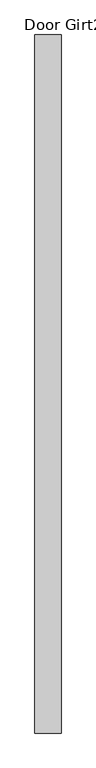
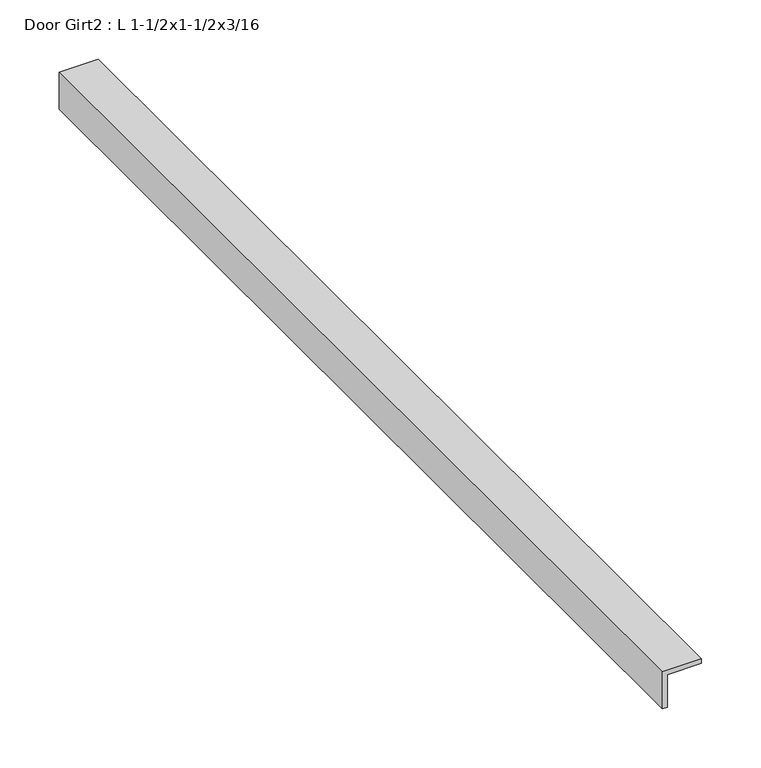
"""IFC4 building model written with IfcOpenShell, lengths in millimetres: proxy geometry, Door Girt2 : L 1-1/2x1-1/2x3/16."""

import ifcopenshell
import ifcopenshell.guid

model = None  # the IFC model being written
_history = None  # IfcOwnerHistory: only IFC2X3 demands one
_inside = {}  # id of a spatial element -> (the spatial element, [elements in it])
_under = {}  # id of a project, library or spatial element -> (it, [spatial elements below it])
_declared = {}  # id of a project -> (the project, [libraries it declares])
_typed = {}  # id of a type object -> (the type object, [elements of that type])
_made_of = {}  # id of a material, layer set ... -> (it, [elements and type objects made of it])


def new_model(schema):
    """Start an empty IFC model of exactly this schema.

    Asked for "IFC4X3", IfcOpenShell would pick the latest addendum, in which some entities
    have other attributes; the version numbers below select the first issue.
    IFC2X3 requires an IfcOwnerHistory on every rooted entity: one is made here for all.
    """
    global model, _history
    if schema == "IFC4X3":
        model = ifcopenshell.file(schema_version=(4, 3, 0, 0))
    else:
        model = ifcopenshell.file(schema=schema)
    _inside.clear()
    _under.clear()
    _declared.clear()
    _typed.clear()
    _made_of.clear()
    _history = None
    if model.schema == "IFC2X3":
        org = make("IfcOrganization", Name="unknown")
        user = make(
            "IfcPersonAndOrganization",
            ThePerson=make("IfcPerson", FamilyName="unknown"),
            TheOrganization=org,
        )
        app = make(
            "IfcApplication",
            ApplicationDeveloper=org,
            Version="unknown",
            ApplicationFullName="unknown",
            ApplicationIdentifier="unknown",
        )
        _history = make(
            "IfcOwnerHistory",
            OwningUser=user,
            OwningApplication=app,
            ChangeAction="ADDED",
            CreationDate=0,
        )
    return model


def make(cls, **values):
    """One entity of the class cls with the attributes given. An attribute that is None is left unset."""
    return model.create_entity(
        cls, **{name: value for name, value in values.items() if value is not None}
    )


def rooted(cls, **values):
    """An entity with a GlobalId (a new one), such as an element, a storey or a relation."""
    return make(cls, GlobalId=ifcopenshell.guid.new(), OwnerHistory=_history, **values)


def si_unit(unit_type, name, prefix=None):
    """IfcSIUnit, for example si_unit("LENGTHUNIT", "METRE", prefix="MILLI")."""
    return make("IfcSIUnit", UnitType=unit_type, Prefix=prefix, Name=name)


def assignment(units):
    """IfcUnitAssignment: the units of a project."""
    return None if units is None else make("IfcUnitAssignment", Units=units)


def point(xyz):
    """IfcCartesianPoint."""
    return None if xyz is None else make("IfcCartesianPoint", Coordinates=xyz)


def direction(xyz):
    """IfcDirection."""
    return None if xyz is None else make("IfcDirection", DirectionRatios=xyz)


def frame(location, z_axis=None, x_axis=None):
    """IfcAxis2Placement3D, a coordinate frame: its origin and axes. An axis left out is left unset."""
    return make(
        "IfcAxis2Placement3D",
        Location=point(location),
        Axis=direction(z_axis),
        RefDirection=direction(x_axis),
    )


def origin():
    """The frame at (0, 0, 0) with its axes left unset."""
    return frame((0.0, 0.0, 0.0))


def place(relative_to, where):
    """IfcLocalPlacement: puts the frame where relative to a parent placement (None: the world)."""
    return make(
        "IfcLocalPlacement", PlacementRelTo=relative_to, RelativePlacement=where
    )


def context(
    kind, dimensions, precision=None, world=None, true_north=None, identifier=None
):
    """IfcGeometricRepresentationContext, for example the 3D "Model" context."""
    return make(
        "IfcGeometricRepresentationContext",
        ContextIdentifier=identifier,
        ContextType=kind,
        CoordinateSpaceDimension=dimensions,
        Precision=precision,
        WorldCoordinateSystem=world,
        TrueNorth=true_north,
    )


def project(units=None, contexts=None):
    """IfcProject with its units and contexts."""
    return rooted(
        "IfcProject",
        Name="project",
        RepresentationContexts=contexts,
        UnitsInContext=assignment(units),
    )


def spatial(cls, under=None, at=None, **own):
    """A site, building, storey or space (cls), placed at a placement, below another one or the project."""
    s = rooted(cls, ObjectPlacement=at, **own)
    if under is not None:
        _under.setdefault(under.id(), (under, []))[1].append(s)
    return s


def polyline(points):
    """IfcPolyline through the points."""
    return make("IfcPolyline", Points=[point(p) for p in points])


def outline(outer, holes=None, kind="AREA"):
    """IfcArbitraryClosedProfileDef: a profile drawn as a closed curve; with holes, ...WithVoids."""
    if holes is None:
        return make("IfcArbitraryClosedProfileDef", ProfileType=kind, OuterCurve=outer)
    return make(
        "IfcArbitraryProfileDefWithVoids",
        ProfileType=kind,
        OuterCurve=outer,
        InnerCurves=holes,
    )


def extrude(swept, where, along, depth):
    """IfcExtrudedAreaSolid: the profile swept, set in the frame where, extruded along a direction by depth."""
    return make(
        "IfcExtrudedAreaSolid",
        SweptArea=swept,
        Position=where,
        ExtrudedDirection=direction(along),
        Depth=depth,
    )


def shape(context_of_items, identifier, shape_type, items):
    """IfcShapeRepresentation: the items that make up one representation, for example the "Body"."""
    return make(
        "IfcShapeRepresentation",
        ContextOfItems=context_of_items,
        RepresentationIdentifier=identifier,
        RepresentationType=shape_type,
        Items=items,
    )


def source(mapping_origin, context_of_items, identifier, shape_type, items):
    """IfcRepresentationMap: a shape defined once, which mapped items show again and again."""
    return make(
        "IfcRepresentationMap",
        MappingOrigin=mapping_origin,
        MappedRepresentation=shape(context_of_items, identifier, shape_type, items),
    )


def transform(
    local_origin,
    x_axis=None,
    y_axis=None,
    z_axis=None,
    scale=None,
    scale2=None,
    scale3=None,
    uniform=True,
):
    """IfcCartesianTransformationOperator3D, or its non-uniform kind. x_axis, y_axis, z_axis: its Axis1, 2, 3."""
    if uniform:
        return make(
            "IfcCartesianTransformationOperator3D",
            Axis1=direction(x_axis),
            Axis2=direction(y_axis),
            LocalOrigin=point(local_origin),
            Scale=scale,
            Axis3=direction(z_axis),
        )
    return make(
        "IfcCartesianTransformationOperator3DnonUniform",
        Axis1=direction(x_axis),
        Axis2=direction(y_axis),
        LocalOrigin=point(local_origin),
        Scale=scale,
        Axis3=direction(z_axis),
        Scale2=scale2,
        Scale3=scale3,
    )


def mapped(mapping_source, mapping_target):
    """IfcMappedItem: shows the shape of a source again, moved by a transform."""
    return make(
        "IfcMappedItem", MappingSource=mapping_source, MappingTarget=mapping_target
    )


def made_of(thing, what):
    """Note that an element or type object is made of a material, layer set ...; save() writes the relation."""
    if what is not None:
        _made_of.setdefault(what.id(), (what, []))[1].append(thing)
    return thing


def element(
    cls,
    number,
    at=None,
    inside=None,
    cuts=None,
    type_object=None,
    material=None,
    context=None,
    identifier="Body",
    shape_type=None,
    held_by="IfcProductDefinitionShape",
    body=None,
    shapes=None,
    **own,
):
    """One element of the class cls, such as IfcWall. Its Tag is "e" and its number.

    at: its placement. inside: the storey or other place that contains it. cuts: it is an
    opening in that element (IfcRelVoidsElement). A single representation is given by context,
    identifier, shape_type and body (its items); several are given by shapes. held_by: the class
    of the entity that holds the representations. save() writes the other relations.
    """
    e = rooted(cls, Tag="e%d" % number, ObjectPlacement=at, **own)
    if body is not None:
        shapes = [shape(context, identifier, shape_type, body)]
    if shapes is not None:
        e.Representation = make(held_by, Representations=shapes)
    if inside is not None:
        _inside.setdefault(inside.id(), (inside, []))[1].append(e)
    if cuts is not None:
        rooted(
            "IfcRelVoidsElement", RelatingBuildingElement=cuts, RelatedOpeningElement=e
        )
    if type_object is not None:
        _typed.setdefault(type_object.id(), (type_object, []))[1].append(e)
    return made_of(e, material)


def aggregate(whole, parts):
    """IfcRelAggregates: a whole, such as a stair, and the parts it consists of."""
    return rooted("IfcRelAggregates", RelatingObject=whole, RelatedObjects=parts)


def save(model, path):
    """Write the relations noted so far, then the file.

    IfcRelAggregates (storeys below a building ...), IfcRelContainedInSpatialStructure (elements
    in a storey), IfcRelDefinesByType, IfcRelAssociatesMaterial and IfcRelDeclares: one each for
    every whole, place, type object, material and project.
    """
    for whole, parts in _under.values():
        aggregate(whole, parts)
    for where, things in _inside.values():
        rooted(
            "IfcRelContainedInSpatialStructure",
            RelatedElements=things,
            RelatingStructure=where,
        )
    for kind, things in _typed.values():
        rooted("IfcRelDefinesByType", RelatedObjects=things, RelatingType=kind)
    for what, things in _made_of.values():
        rooted("IfcRelAssociatesMaterial", RelatedObjects=things, RelatingMaterial=what)
    for by, libraries in _declared.values():
        rooted("IfcRelDeclares", RelatingContext=by, RelatedDefinitions=libraries)
    model.write(path)


def door_girt2_l_1_1_2x1_1_2x3_16_4184d8b8(model_context):
    return source(origin(), model_context, "Body", "SweptSolid", [
        extrude(outline(polyline([(812.8, 587403.9934739), (812.8, 587365.8934739), (774.7, 587365.8934739), (774.7, 587370.6559739), (808.0375, 587370.6559739), (808.0375, 587403.9934739), (812.8, 587403.9934739)])), frame((0.0, -535163.4663841, 0.0), z_axis=(0.0, 1.0, 0.0), x_axis=(0.0, 0.0, 1.0)), (0.0, 0.0, 1.0), 1017.5875),
    ])


if __name__ == "__main__":
    model = new_model("IFC4")
    model_context = context("Model", 3, world=origin())
    ifc_project = project(units=[si_unit("LENGTHUNIT", "METRE", prefix="MILLI")], contexts=[model_context])
    site = spatial("IfcSite", under=ifc_project)
    building = spatial("IfcBuilding", under=site)
    placement = place(None, origin())
    door_girt2_l_1_1_2x1_1_2x3_16_shape = door_girt2_l_1_1_2x1_1_2x3_16_4184d8b8(model_context)
    element("IfcBuildingElementProxy", 1, Name="Door Girt2 : L 1-1/2x1-1/2x3/16", ObjectType="Door Girt2 : L 1-1/2x1-1/2x3/16", at=placement, inside=building, context=model_context, shape_type="MappedRepresentation", body=[
        mapped(door_girt2_l_1_1_2x1_1_2x3_16_shape, transform((0.0, 0.0, 0.0), x_axis=(1.0, 0.0, 0.0), y_axis=(0.0, 1.0, 0.0), z_axis=(0.0, 0.0, 1.0))),
    ])
    save(model, "model.ifc")

# Revit data of these elements
# Element 1 (IfcBuildingElementProxy, "Door Girt2 : L 1-1/2x1-1/2x3/16")
#   Materials on its faces: "1-1/2\"X1-1/2\" GALV. STL L"
# Materials
#   "1-1/2\"X1-1/2\" GALV. STL L": class "Generic", colour RGB 211 211 207, transparency 0, Cost = 0
